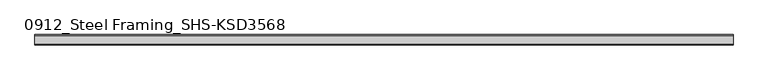
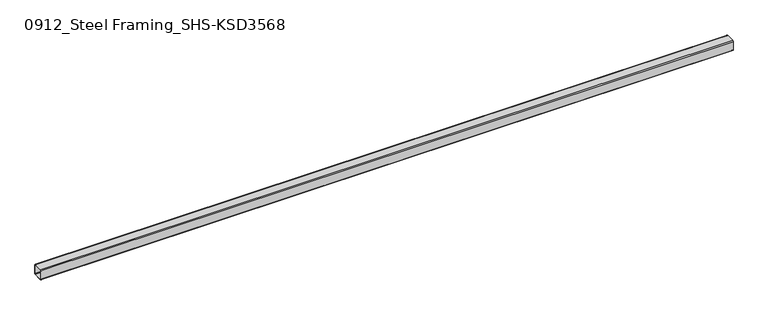
"""IFC4 building model written with IfcOpenShell, lengths in millimetres: beam geometry, 0912_Steel Framing_SHS-KSD3568 : H_SB_ASB_SHS-150x150x6."""

from ifc_helpers import new_model, si_unit, point, frame, frame_2d, origin, place, context, project, spatial, polyline, circle_curve, trimmed, segment, composite_curve, outline, extrude, source, transform, mapped, element, save


def beam_0912_steel_framing_shs_ksd3568_ac36583f(model_context):
    return source(origin(), model_context, "Body", "SweptSolid", [
        extrude(outline(composite_curve([segment(polyline([(75.0, 63.0), (75.0, -63.0)]), True, "CONTINUOUS"), segment(trimmed(circle_curve(frame_2d((63.0, -63.0)), 12.0), [point((75.0, -63.0))], [point((63.0, -75.0))], False, "CARTESIAN"), True, "CONTINUOUS"), segment(polyline([(63.0, -75.0), (-63.0, -75.0)]), True, "CONTINUOUS"), segment(trimmed(circle_curve(frame_2d((-63.0, -63.0)), 12.0), [point((-63.0, -75.0))], [point((-75.0, -63.0))], False, "CARTESIAN"), True, "CONTINUOUS"), segment(polyline([(-75.0, -63.0), (-75.0, 63.0)]), True, "CONTINUOUS"), segment(trimmed(circle_curve(frame_2d((-63.0, 63.0)), 12.0), [point((-75.0, 63.0))], [point((-63.0, 75.0))], False, "CARTESIAN"), True, "CONTINUOUS"), segment(polyline([(-63.0, 75.0), (63.0, 75.0)]), True, "CONTINUOUS"), segment(trimmed(circle_curve(frame_2d((63.0, 63.0)), 12.0), [point((63.0, 75.0))], [point((75.0, 63.0))], False, "CARTESIAN"), True, "CONTINUOUS")], self_intersect=False), holes=[composite_curve([segment(trimmed(circle_curve(frame_2d((-63.0, 63.0)), 6.0), [point((-63.0, 69.0))], [point((-69.0, 63.0))], True, "CARTESIAN"), True, "CONTINUOUS"), segment(polyline([(-69.0, 63.0), (-69.0, -63.0)]), True, "CONTINUOUS"), segment(trimmed(circle_curve(frame_2d((-63.0, -63.0)), 6.0), [point((-69.0, -63.0))], [point((-63.0, -69.0))], True, "CARTESIAN"), True, "CONTINUOUS"), segment(polyline([(-63.0, -69.0), (63.0, -69.0)]), True, "CONTINUOUS"), segment(trimmed(circle_curve(frame_2d((63.0, -63.0)), 6.0), [point((63.0, -69.0))], [point((69.0, -63.0))], True, "CARTESIAN"), True, "CONTINUOUS"), segment(polyline([(69.0, -63.0), (69.0, 63.0)]), True, "CONTINUOUS"), segment(trimmed(circle_curve(frame_2d((63.0, 63.0)), 6.0), [point((69.0, 63.0))], [point((63.0, 69.0))], True, "CARTESIAN"), True, "CONTINUOUS"), segment(polyline([(63.0, 69.0), (-63.0, 69.0)]), True, "CONTINUOUS")], self_intersect=False)]), frame((-4882.3, 0.0, 0.0), z_axis=(1.0, 0.0, 0.0), x_axis=(0.0, 1.0, 0.0)), (0.0, 0.0, 1.0), 9917.3),
    ])


if __name__ == "__main__":
    model = new_model("IFC4")
    model_context = context("Model", 3, world=origin())
    ifc_project = project(units=[si_unit("LENGTHUNIT", "METRE", prefix="MILLI")], contexts=[model_context])
    site = spatial("IfcSite", under=ifc_project)
    building = spatial("IfcBuilding", under=site)
    placement = place(None, origin())
    beam_0912_steel_framing_shs_ksd3568_shape = beam_0912_steel_framing_shs_ksd3568_ac36583f(model_context)
    element("IfcBeam", 1, ObjectType="0912_Steel Framing_SHS-KSD3568 : H_SB_ASB_SHS-150x150x6", at=placement, inside=building, context=model_context, shape_type="MappedRepresentation", body=[
        mapped(beam_0912_steel_framing_shs_ksd3568_shape, transform((0.0, 0.0, 0.0), x_axis=(1.0, 0.0, 0.0), y_axis=(0.0, 1.0, 0.0), z_axis=(0.0, 0.0, 1.0))),
    ])
    save(model, "model.ifc")

# Revit data of these elements
# Type "0912_Steel Framing_SHS-KSD3568 : H_SB_ASB_SHS-150x150x6"
#   H_WM Code_1 = "S01AA002-00001 | Main Steel Structure Fabrication Work | Shelter/Building | Medium Steel - Standard (90KG/M>Weight≥30KG/M) | Material: (   )"
#   H_WM Code_2 = "S03AA028-00001 | Main Steel Structure Erection Work | Shelter/Building | Medium Steel (90KG/M>Weight≥30KG/M) | Material: (   )"
#   H_WM Code_3 = "S01AA010-00001 | Main Steel Structure Fabrication Work | Shelter/Building | Steel Painting/Coating | for Non-Fireproofed Steel Surface, Surface Preparation, Primer, Second & Final Coat | Material: (   )"
#   H_Q'ty Cal Type Tag = "SB-Q2"
#   Perimeter = 0.60 m²/m
#   Nominal Weight = 26.40 kgf/m
#   Length [instance default] = 1.0000 m
#   b = 0.1500 m
#   h = 0.1500 m
#   tr = 0.0120 m
#   t = 0.0060 m
#   A = 28.36 m²
#   Structural Material [instance default] = Steel, 45-345
# Element 1 (IfcBeam, "0912_Steel Framing_SHS-KSD3568 : H_SB_ASB_SHS-150x150x6")
#   Structural Material = none
# Materials
#   "Steel, 45-345": class "Metal", colour RGB 189 187 185, transparency 0, Description = "Steel 345 MPa", Cost = 0
